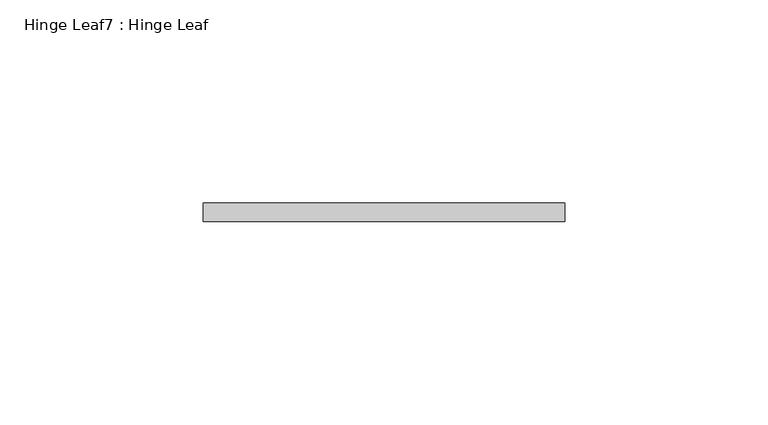
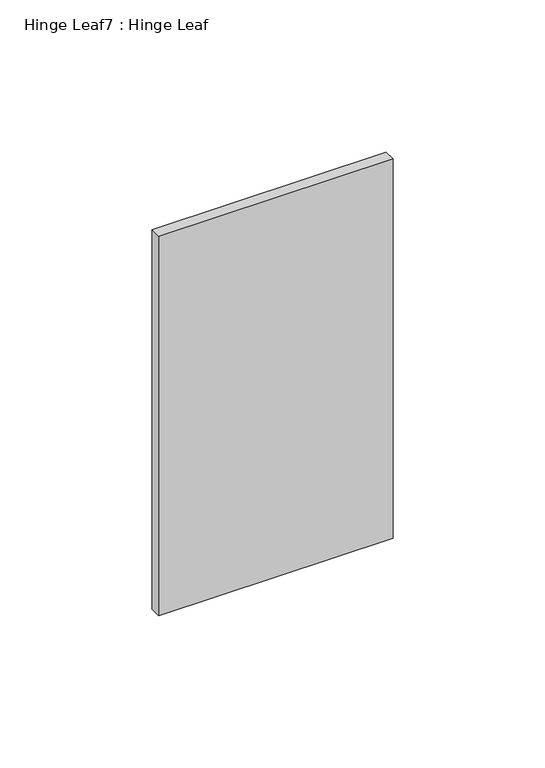
"""IFC4 building model written with IfcOpenShell, lengths in millimetres: proxy geometry, Hinge Leaf7 : Hinge Leaf."""

from ifc_helpers import new_model, si_unit, frame, origin, place, context, project, spatial, polyline, outline, extrude, source, transform, mapped, element, save


def hinge_leaf7_hinge_leaf_106c3047(model_context):
    return source(origin(), model_context, "Body", "SweptSolid", [
        extrude(outline(polyline([(587327.7934739, -533988.7163841), (587327.7934739, -533984.1443841), (587416.6934739, -533984.1443841), (587416.6934739, -533988.7163841), (587327.7934739, -533988.7163841)])), frame((0.0, 0.0, 311.15), z_axis=(0.0, 0.0, 1.0), x_axis=(1.0, 0.0, 0.0)), (0.0, 0.0, 1.0), 152.4),
    ])


if __name__ == "__main__":
    model = new_model("IFC4")
    model_context = context("Model", 3, world=origin())
    ifc_project = project(units=[si_unit("LENGTHUNIT", "METRE", prefix="MILLI")], contexts=[model_context])
    site = spatial("IfcSite", under=ifc_project)
    building = spatial("IfcBuilding", under=site)
    placement = place(None, origin())
    hinge_leaf7_hinge_leaf_shape = hinge_leaf7_hinge_leaf_106c3047(model_context)
    element("IfcBuildingElementProxy", 1, Name="Hinge Leaf7 : Hinge Leaf", ObjectType="Hinge Leaf7 : Hinge Leaf", at=placement, inside=building, context=model_context, shape_type="MappedRepresentation", body=[
        mapped(hinge_leaf7_hinge_leaf_shape, transform((0.0, 0.0, 0.0), x_axis=(1.0, 0.0, 0.0), y_axis=(0.0, 1.0, 0.0), z_axis=(0.0, 0.0, 1.0))),
    ])
    save(model, "model.ifc")

# Revit data of these elements
# Element 1 (IfcBuildingElementProxy, "Hinge Leaf7 : Hinge Leaf")
#   Materials on its faces: "6\"X6\" WELD-ON STL BUTT HINGE"
# Materials
#   "6\"X6\" WELD-ON STL BUTT HINGE": class "Metal", colour RGB 189 187 185, transparency 0, Description = "Carbon steel", Cost = 0
